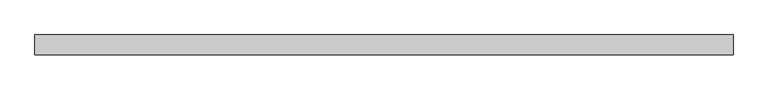
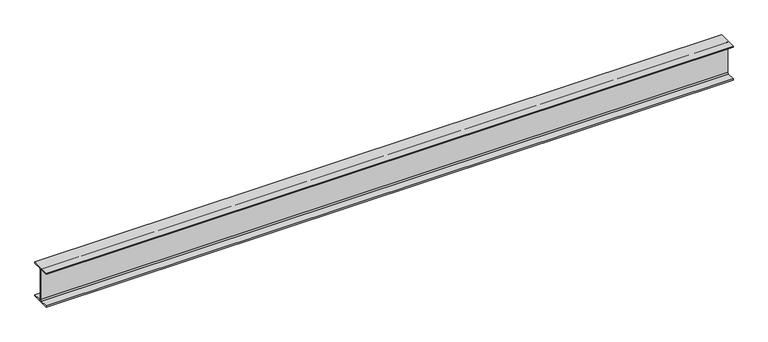
"""IFC4 building model written with IfcOpenShell, lengths in millimetres: beam geometry, Old_Steel Beam_H-KSD3502 : H_SB_ASB_H-350×175x7x11."""

from ifc_helpers import new_model, si_unit, point, frame, frame_2d, origin, place, context, project, spatial, polyline, circle_curve, trimmed, segment, composite_curve, outline, extrude, source, transform, mapped, element, save


def beam_d1923d8f(model_context):
    return source(origin(), model_context, "Body", "SweptSolid", [
        extrude(outline(composite_curve([segment(polyline([(82.5, -141.5), (82.5, -151.7), (-82.5, -151.7), (-82.5, -141.5), (-11.9, -141.5)]), True, "CONTINUOUS"), segment(trimmed(circle_curve(frame_2d((-11.9, -132.6)), 8.9), [point((-11.9, -141.5))], [point((-3.0, -132.6))], True, "CARTESIAN"), True, "CONTINUOUS"), segment(polyline([(-3.0, -132.6), (-3.0, 132.6)]), True, "CONTINUOUS"), segment(trimmed(circle_curve(frame_2d((-11.9, 132.6)), 8.9), [point((-3.0, 132.6))], [point((-11.9, 141.5))], True, "CARTESIAN"), True, "CONTINUOUS"), segment(polyline([(-11.9, 141.5), (-82.5, 141.5), (-82.5, 151.7), (82.5, 151.7), (82.5, 141.5), (11.9, 141.5)]), True, "CONTINUOUS"), segment(trimmed(circle_curve(frame_2d((11.9, 132.6)), 8.9), [point((11.9, 141.5))], [point((3.0, 132.6))], True, "CARTESIAN"), True, "CONTINUOUS"), segment(polyline([(3.0, 132.6), (3.0, -132.6)]), True, "CONTINUOUS"), segment(trimmed(circle_curve(frame_2d((11.9, -132.6)), 8.9), [point((3.0, -132.6))], [point((11.9, -141.5))], True, "CARTESIAN"), True, "CONTINUOUS"), segment(polyline([(11.9, -141.5), (82.5, -141.5)]), True, "CONTINUOUS")], self_intersect=False)), frame((-2912.1972294, 0.0, 0.0), z_axis=(1.0, 0.0, 0.0), x_axis=(0.0, 1.0, 0.0)), (0.0, 0.0, 1.0), 5810.2298939),
    ])


if __name__ == "__main__":
    model = new_model("IFC4")
    model_context = context("Model", 3, world=origin())
    ifc_project = project(units=[si_unit("LENGTHUNIT", "METRE", prefix="MILLI")], contexts=[model_context])
    site = spatial("IfcSite", under=ifc_project)
    building = spatial("IfcBuilding", under=site)
    placement = place(None, origin())
    beam_shape = beam_d1923d8f(model_context)
    element("IfcBeam", 1, ObjectType="Old_Steel Beam_H-KSD3502 : H_SB_ASB_H-350×175x7x11", at=placement, inside=building, context=model_context, shape_type="MappedRepresentation", body=[
        mapped(beam_shape, transform((0.0, 0.0, 0.0), x_axis=(1.0, 0.0, 0.0), y_axis=(0.0, 1.0, 0.0), z_axis=(0.0, 0.0, 1.0))),
    ])
    save(model, "model.ifc")

# Revit data of these elements
# Type "Old_Steel Beam_H-KSD3502 : H_SB_ASB_H-350×175x7x11"
#   Width = 17.5 cm
#   Web Thickness = 0.7 cm
#   Web Fillet = 1.4 cm
#   Warping Constant = 282290.0 cm⁶
#   Torsional Moment of Inertia = 19.4042 cm⁴
#   Torsional Modulus = 1.0 cm³
#   Section Area = 63.14 cm²
#   Plastic Modulus weak axis = 174.0 cm³
#   Plastic Modulus strong axis = 868.0 cm³
#   Perimeter = 1.36 m²/m
#   Nominal Weight = 49.60 kgf/m
#   Moment of Inertia weak axis = 984.00 cm⁴
#   Moment of Inertia strong axis = 13600.00 cm⁴
#   Height = 35.0 cm
#   Flange Thickness = 1.1 cm
#   Elastic Modulus weak axis = 112.0 cm³
#   Elastic Modulus strong axis = 775.0 cm³
#   Centroid Vertical = 17.5 cm
#   Centroid Horizontal = 8.75 cm
#   Length [instance default] = 1.5240 m
#   Structural Material [instance default] = Steel, 45-345
#   Assembly Code = ""
# Element 1 (IfcBeam, "Old_Steel Beam_H-KSD3502 : H_SB_ASB_H-350×175x7x11")
#   Structural Material = none
# Materials
#   "Steel, 45-345": class "Metal", colour RGB 189 187 185, transparency 0, Description = "Steel 345 MPa", Cost = 0
